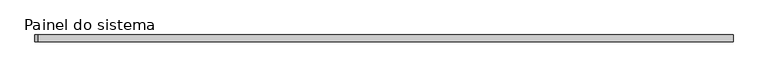
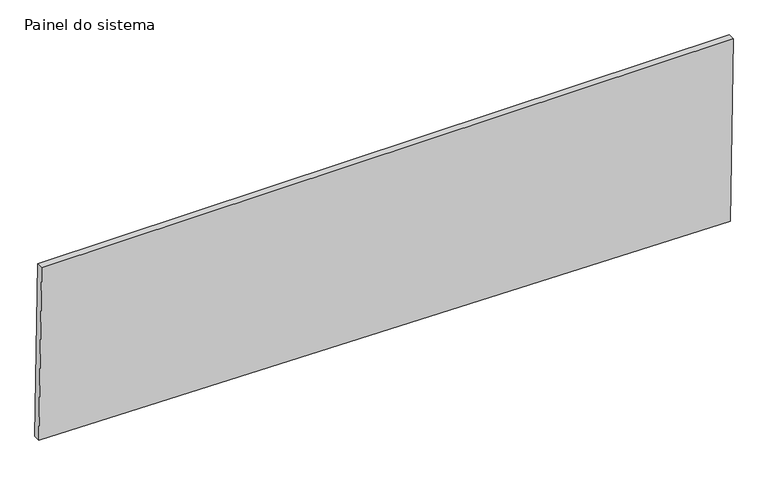
"""IFC4 building model written with IfcOpenShell, lengths in millimetres: plate geometry, Painel do sistema : Envidraçado."""

from ifc_helpers import new_model, si_unit, frame, origin, place, context, project, spatial, polyline, outline, extrude, source, transform, mapped, element, save


def painel_do_sistema_3dd8ea3f(model_context):
    return source(origin(), model_context, "Body", "SweptSolid", [
        extrude(outline(polyline([(38.3128408, -1278.9812381), (0.0, 1268.3596124), (706.209735, 1278.9812381), (706.209735, -1268.9358501), (38.3128408, -1278.9812381)])), frame((0.0, 24.5, 0.0), z_axis=(0.0, 1.0, 0.0), x_axis=(0.0, 0.0, 1.0)), (0.0, 0.0, 1.0), 25.0),
    ])


if __name__ == "__main__":
    model = new_model("IFC4")
    model_context = context("Model", 3, world=origin())
    ifc_project = project(units=[si_unit("LENGTHUNIT", "METRE", prefix="MILLI")], contexts=[model_context])
    site = spatial("IfcSite", under=ifc_project)
    building = spatial("IfcBuilding", under=site)
    placement = place(None, origin())
    painel_do_sistema_shape = painel_do_sistema_3dd8ea3f(model_context)
    element("IfcPlate", 1, ObjectType="Painel do sistema : Envidraçado", at=placement, inside=building, context=model_context, shape_type="MappedRepresentation", body=[
        mapped(painel_do_sistema_shape, transform((0.0, 0.0, 0.0), x_axis=(1.0, 0.0, 0.0), y_axis=(0.0, 1.0, 0.0), z_axis=(0.0, 0.0, 1.0))),
    ])
    save(model, "model.ifc")

# Revit data of these elements
# Type "Painel do sistema : Envidraçado"
#   Construction Type Id = "GSP4R"
#   Analytic Construction = "Vidraça única Pilkington 1/8 pol"
#   Visual Light Transmittance = 0.9
#   Solar Heat Gain Coefficient = 0.86
#   Heat Transfer Coefficient (U) = 6.7069 W/(m²·K)
# Element 1 (IfcPlate, "Painel do sistema : Envidraçado")
#   Materials on its faces: "Vidro"
# Materials
#   "Vidro": class "Vidro", colour RGB 0 128 192, transparency 0.9, Description = "Vidro de sílica", Cost = 0
